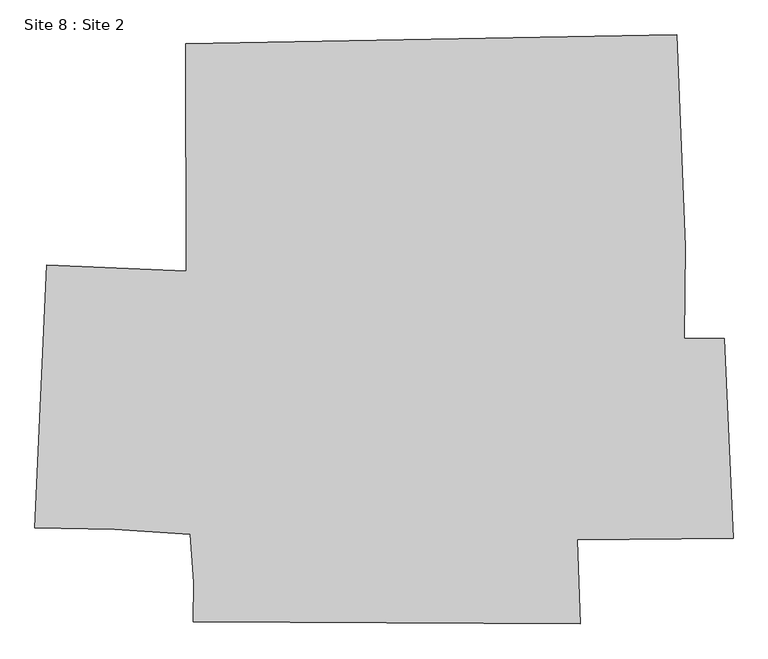
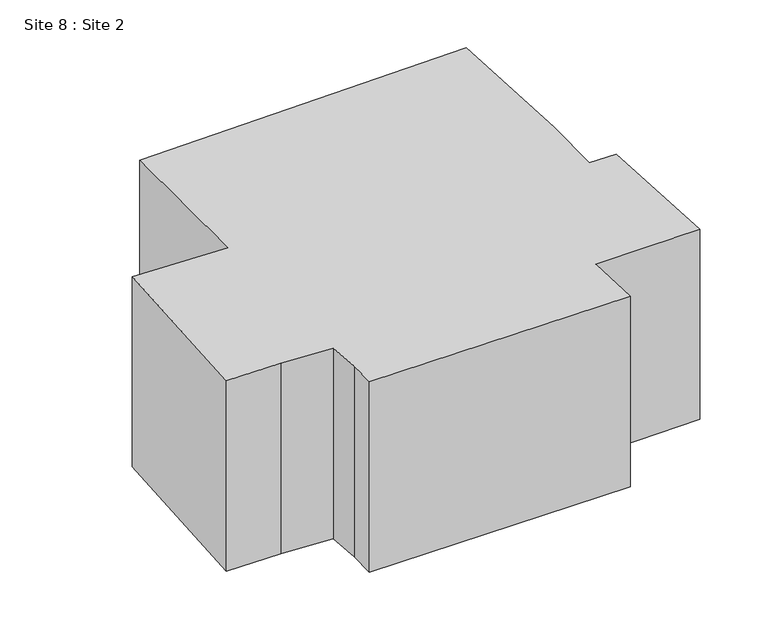
"""IFC4 building model written with IfcOpenShell, lengths in millimetres: geographic element geometry, Site 8 : Site 2."""

import ifcopenshell
import ifcopenshell.guid

model = None  # the IFC model being written
_history = None  # IfcOwnerHistory: only IFC2X3 demands one
_inside = {}  # id of a spatial element -> (the spatial element, [elements in it])
_under = {}  # id of a project, library or spatial element -> (it, [spatial elements below it])
_declared = {}  # id of a project -> (the project, [libraries it declares])
_typed = {}  # id of a type object -> (the type object, [elements of that type])
_made_of = {}  # id of a material, layer set ... -> (it, [elements and type objects made of it])


def new_model(schema):
    """Start an empty IFC model of exactly this schema.

    Asked for "IFC4X3", IfcOpenShell would pick the latest addendum, in which some entities
    have other attributes; the version numbers below select the first issue.
    IFC2X3 requires an IfcOwnerHistory on every rooted entity: one is made here for all.
    """
    global model, _history
    if schema == "IFC4X3":
        model = ifcopenshell.file(schema_version=(4, 3, 0, 0))
    else:
        model = ifcopenshell.file(schema=schema)
    _inside.clear()
    _under.clear()
    _declared.clear()
    _typed.clear()
    _made_of.clear()
    _history = None
    if model.schema == "IFC2X3":
        org = make("IfcOrganization", Name="unknown")
        user = make(
            "IfcPersonAndOrganization",
            ThePerson=make("IfcPerson", FamilyName="unknown"),
            TheOrganization=org,
        )
        app = make(
            "IfcApplication",
            ApplicationDeveloper=org,
            Version="unknown",
            ApplicationFullName="unknown",
            ApplicationIdentifier="unknown",
        )
        _history = make(
            "IfcOwnerHistory",
            OwningUser=user,
            OwningApplication=app,
            ChangeAction="ADDED",
            CreationDate=0,
        )
    return model


def make(cls, **values):
    """One entity of the class cls with the attributes given. An attribute that is None is left unset."""
    return model.create_entity(
        cls, **{name: value for name, value in values.items() if value is not None}
    )


def rooted(cls, **values):
    """An entity with a GlobalId (a new one), such as an element, a storey or a relation."""
    return make(cls, GlobalId=ifcopenshell.guid.new(), OwnerHistory=_history, **values)


def si_unit(unit_type, name, prefix=None):
    """IfcSIUnit, for example si_unit("LENGTHUNIT", "METRE", prefix="MILLI")."""
    return make("IfcSIUnit", UnitType=unit_type, Prefix=prefix, Name=name)


def assignment(units):
    """IfcUnitAssignment: the units of a project."""
    return None if units is None else make("IfcUnitAssignment", Units=units)


def point(xyz):
    """IfcCartesianPoint."""
    return None if xyz is None else make("IfcCartesianPoint", Coordinates=xyz)


def direction(xyz):
    """IfcDirection."""
    return None if xyz is None else make("IfcDirection", DirectionRatios=xyz)


def frame(location, z_axis=None, x_axis=None):
    """IfcAxis2Placement3D, a coordinate frame: its origin and axes. An axis left out is left unset."""
    return make(
        "IfcAxis2Placement3D",
        Location=point(location),
        Axis=direction(z_axis),
        RefDirection=direction(x_axis),
    )


def origin():
    """The frame at (0, 0, 0) with its axes left unset."""
    return frame((0.0, 0.0, 0.0))


def place(relative_to, where):
    """IfcLocalPlacement: puts the frame where relative to a parent placement (None: the world)."""
    return make(
        "IfcLocalPlacement", PlacementRelTo=relative_to, RelativePlacement=where
    )


def context(
    kind, dimensions, precision=None, world=None, true_north=None, identifier=None
):
    """IfcGeometricRepresentationContext, for example the 3D "Model" context."""
    return make(
        "IfcGeometricRepresentationContext",
        ContextIdentifier=identifier,
        ContextType=kind,
        CoordinateSpaceDimension=dimensions,
        Precision=precision,
        WorldCoordinateSystem=world,
        TrueNorth=true_north,
    )


def project(units=None, contexts=None):
    """IfcProject with its units and contexts."""
    return rooted(
        "IfcProject",
        Name="project",
        RepresentationContexts=contexts,
        UnitsInContext=assignment(units),
    )


def spatial(cls, under=None, at=None, **own):
    """A site, building, storey or space (cls), placed at a placement, below another one or the project."""
    s = rooted(cls, ObjectPlacement=at, **own)
    if under is not None:
        _under.setdefault(under.id(), (under, []))[1].append(s)
    return s


def polyline(points):
    """IfcPolyline through the points."""
    return make("IfcPolyline", Points=[point(p) for p in points])


def outline(outer, holes=None, kind="AREA"):
    """IfcArbitraryClosedProfileDef: a profile drawn as a closed curve; with holes, ...WithVoids."""
    if holes is None:
        return make("IfcArbitraryClosedProfileDef", ProfileType=kind, OuterCurve=outer)
    return make(
        "IfcArbitraryProfileDefWithVoids",
        ProfileType=kind,
        OuterCurve=outer,
        InnerCurves=holes,
    )


def extrude(swept, where, along, depth):
    """IfcExtrudedAreaSolid: the profile swept, set in the frame where, extruded along a direction by depth."""
    return make(
        "IfcExtrudedAreaSolid",
        SweptArea=swept,
        Position=where,
        ExtrudedDirection=direction(along),
        Depth=depth,
    )


def shape(context_of_items, identifier, shape_type, items):
    """IfcShapeRepresentation: the items that make up one representation, for example the "Body"."""
    return make(
        "IfcShapeRepresentation",
        ContextOfItems=context_of_items,
        RepresentationIdentifier=identifier,
        RepresentationType=shape_type,
        Items=items,
    )


def source(mapping_origin, context_of_items, identifier, shape_type, items):
    """IfcRepresentationMap: a shape defined once, which mapped items show again and again."""
    return make(
        "IfcRepresentationMap",
        MappingOrigin=mapping_origin,
        MappedRepresentation=shape(context_of_items, identifier, shape_type, items),
    )


def transform(
    local_origin,
    x_axis=None,
    y_axis=None,
    z_axis=None,
    scale=None,
    scale2=None,
    scale3=None,
    uniform=True,
):
    """IfcCartesianTransformationOperator3D, or its non-uniform kind. x_axis, y_axis, z_axis: its Axis1, 2, 3."""
    if uniform:
        return make(
            "IfcCartesianTransformationOperator3D",
            Axis1=direction(x_axis),
            Axis2=direction(y_axis),
            LocalOrigin=point(local_origin),
            Scale=scale,
            Axis3=direction(z_axis),
        )
    return make(
        "IfcCartesianTransformationOperator3DnonUniform",
        Axis1=direction(x_axis),
        Axis2=direction(y_axis),
        LocalOrigin=point(local_origin),
        Scale=scale,
        Axis3=direction(z_axis),
        Scale2=scale2,
        Scale3=scale3,
    )


def mapped(mapping_source, mapping_target):
    """IfcMappedItem: shows the shape of a source again, moved by a transform."""
    return make(
        "IfcMappedItem", MappingSource=mapping_source, MappingTarget=mapping_target
    )


def made_of(thing, what):
    """Note that an element or type object is made of a material, layer set ...; save() writes the relation."""
    if what is not None:
        _made_of.setdefault(what.id(), (what, []))[1].append(thing)
    return thing


def element(
    cls,
    number,
    at=None,
    inside=None,
    cuts=None,
    type_object=None,
    material=None,
    context=None,
    identifier="Body",
    shape_type=None,
    held_by="IfcProductDefinitionShape",
    body=None,
    shapes=None,
    **own,
):
    """One element of the class cls, such as IfcWall. Its Tag is "e" and its number.

    at: its placement. inside: the storey or other place that contains it. cuts: it is an
    opening in that element (IfcRelVoidsElement). A single representation is given by context,
    identifier, shape_type and body (its items); several are given by shapes. held_by: the class
    of the entity that holds the representations. save() writes the other relations.
    """
    e = rooted(cls, Tag="e%d" % number, ObjectPlacement=at, **own)
    if body is not None:
        shapes = [shape(context, identifier, shape_type, body)]
    if shapes is not None:
        e.Representation = make(held_by, Representations=shapes)
    if inside is not None:
        _inside.setdefault(inside.id(), (inside, []))[1].append(e)
    if cuts is not None:
        rooted(
            "IfcRelVoidsElement", RelatingBuildingElement=cuts, RelatedOpeningElement=e
        )
    if type_object is not None:
        _typed.setdefault(type_object.id(), (type_object, []))[1].append(e)
    return made_of(e, material)


def aggregate(whole, parts):
    """IfcRelAggregates: a whole, such as a stair, and the parts it consists of."""
    return rooted("IfcRelAggregates", RelatingObject=whole, RelatedObjects=parts)


def save(model, path):
    """Write the relations noted so far, then the file.

    IfcRelAggregates (storeys below a building ...), IfcRelContainedInSpatialStructure (elements
    in a storey), IfcRelDefinesByType, IfcRelAssociatesMaterial and IfcRelDeclares: one each for
    every whole, place, type object, material and project.
    """
    for whole, parts in _under.values():
        aggregate(whole, parts)
    for where, things in _inside.values():
        rooted(
            "IfcRelContainedInSpatialStructure",
            RelatedElements=things,
            RelatingStructure=where,
        )
    for kind, things in _typed.values():
        rooted("IfcRelDefinesByType", RelatedObjects=things, RelatingType=kind)
    for what, things in _made_of.values():
        rooted("IfcRelAssociatesMaterial", RelatedObjects=things, RelatingMaterial=what)
    for by, libraries in _declared.values():
        rooted("IfcRelDeclares", RelatingContext=by, RelatedDefinitions=libraries)
    model.write(path)


def site_8_site_2_3ba1f17e(model_context):
    return source(origin(), model_context, "Body", "SweptSolid", [
        extrude(outline(polyline([(17136.7272759, 29780.0507186), (18152.6239295, 29765.3331737), (18383.8030411, 24681.5193473), (14420.3487659, 24637.3304383), (14491.0298199, 22502.5290813), (4635.3952714, 22543.7016386), (4650.1124484, 23559.5728954), (4566.1817023, 24780.0901826), (2637.4557041, 24909.6405578), (605.6708625, 24939.075525), (905.9833281, 31640.9246511), (4460.1371995, 31487.8263022), (4442.438596, 37279.8065116), (16943.8128244, 37505.1298127), (17170.576783, 32116.5546092), (17136.7272759, 29780.0507186)])), frame((0.0, 0.0, 266395.2), z_axis=(0.0, 0.0, 1.0), x_axis=(1.0, 0.0, 0.0)), (0.0, 0.0, 1.0), 7620.0),
    ])


if __name__ == "__main__":
    model = new_model("IFC4")
    model_context = context("Model", 3, world=origin())
    ifc_project = project(units=[si_unit("LENGTHUNIT", "METRE", prefix="MILLI")], contexts=[model_context])
    site = spatial("IfcSite", under=ifc_project)
    building = spatial("IfcBuilding", under=site)
    placement = place(None, origin())
    site_8_site_2_shape = site_8_site_2_3ba1f17e(model_context)
    element("IfcGeographicElement", 1, ObjectType="Site 8 : Site 2", at=placement, inside=building, context=model_context, shape_type="MappedRepresentation", body=[
        mapped(site_8_site_2_shape, transform((0.0, 0.0, 0.0), x_axis=(1.0, 0.0, 0.0), y_axis=(0.0, 1.0, 0.0), z_axis=(0.0, 0.0, 1.0))),
    ])
    save(model, "model.ifc")

# Revit data of these elements
# Element 1 (IfcGeographicElement, "Site 8 : Site 2")
#   Materials on its faces: "EXISTING BUILDING"
# Materials
#   "EXISTING BUILDING": class "Generic", colour RGB 120 120 120, transparency 0, Cost = 0
